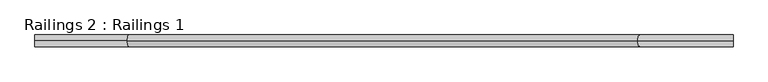
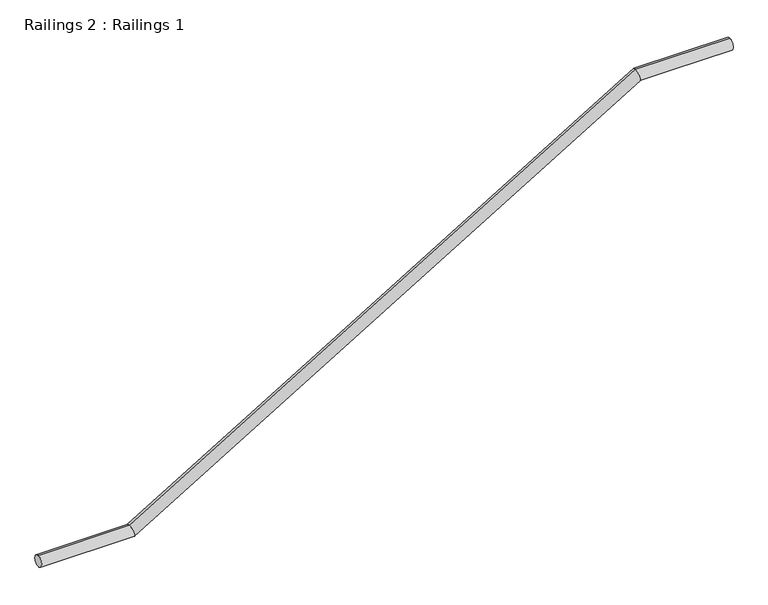
"""IFC4 building model written with IfcOpenShell, lengths in millimetres: railing geometry, Railings 2 : Railings 1."""

import ifcopenshell
import ifcopenshell.guid

model = None  # the IFC model being written
_history = None  # IfcOwnerHistory: only IFC2X3 demands one
_inside = {}  # id of a spatial element -> (the spatial element, [elements in it])
_under = {}  # id of a project, library or spatial element -> (it, [spatial elements below it])
_declared = {}  # id of a project -> (the project, [libraries it declares])
_typed = {}  # id of a type object -> (the type object, [elements of that type])
_made_of = {}  # id of a material, layer set ... -> (it, [elements and type objects made of it])


def new_model(schema):
    """Start an empty IFC model of exactly this schema.

    Asked for "IFC4X3", IfcOpenShell would pick the latest addendum, in which some entities
    have other attributes; the version numbers below select the first issue.
    IFC2X3 requires an IfcOwnerHistory on every rooted entity: one is made here for all.
    """
    global model, _history
    if schema == "IFC4X3":
        model = ifcopenshell.file(schema_version=(4, 3, 0, 0))
    else:
        model = ifcopenshell.file(schema=schema)
    _inside.clear()
    _under.clear()
    _declared.clear()
    _typed.clear()
    _made_of.clear()
    _history = None
    if model.schema == "IFC2X3":
        org = make("IfcOrganization", Name="unknown")
        user = make(
            "IfcPersonAndOrganization",
            ThePerson=make("IfcPerson", FamilyName="unknown"),
            TheOrganization=org,
        )
        app = make(
            "IfcApplication",
            ApplicationDeveloper=org,
            Version="unknown",
            ApplicationFullName="unknown",
            ApplicationIdentifier="unknown",
        )
        _history = make(
            "IfcOwnerHistory",
            OwningUser=user,
            OwningApplication=app,
            ChangeAction="ADDED",
            CreationDate=0,
        )
    return model


def make(cls, **values):
    """One entity of the class cls with the attributes given. An attribute that is None is left unset."""
    return model.create_entity(
        cls, **{name: value for name, value in values.items() if value is not None}
    )


def rooted(cls, **values):
    """An entity with a GlobalId (a new one), such as an element, a storey or a relation."""
    return make(cls, GlobalId=ifcopenshell.guid.new(), OwnerHistory=_history, **values)


def si_unit(unit_type, name, prefix=None):
    """IfcSIUnit, for example si_unit("LENGTHUNIT", "METRE", prefix="MILLI")."""
    return make("IfcSIUnit", UnitType=unit_type, Prefix=prefix, Name=name)


def assignment(units):
    """IfcUnitAssignment: the units of a project."""
    return None if units is None else make("IfcUnitAssignment", Units=units)


def point(xyz):
    """IfcCartesianPoint."""
    return None if xyz is None else make("IfcCartesianPoint", Coordinates=xyz)


def direction(xyz):
    """IfcDirection."""
    return None if xyz is None else make("IfcDirection", DirectionRatios=xyz)


def frame(location, z_axis=None, x_axis=None):
    """IfcAxis2Placement3D, a coordinate frame: its origin and axes. An axis left out is left unset."""
    return make(
        "IfcAxis2Placement3D",
        Location=point(location),
        Axis=direction(z_axis),
        RefDirection=direction(x_axis),
    )


def origin():
    """The frame at (0, 0, 0) with its axes left unset."""
    return frame((0.0, 0.0, 0.0))


def place(relative_to, where):
    """IfcLocalPlacement: puts the frame where relative to a parent placement (None: the world)."""
    return make(
        "IfcLocalPlacement", PlacementRelTo=relative_to, RelativePlacement=where
    )


def context(
    kind, dimensions, precision=None, world=None, true_north=None, identifier=None
):
    """IfcGeometricRepresentationContext, for example the 3D "Model" context."""
    return make(
        "IfcGeometricRepresentationContext",
        ContextIdentifier=identifier,
        ContextType=kind,
        CoordinateSpaceDimension=dimensions,
        Precision=precision,
        WorldCoordinateSystem=world,
        TrueNorth=true_north,
    )


def project(units=None, contexts=None):
    """IfcProject with its units and contexts."""
    return rooted(
        "IfcProject",
        Name="project",
        RepresentationContexts=contexts,
        UnitsInContext=assignment(units),
    )


def spatial(cls, under=None, at=None, **own):
    """A site, building, storey or space (cls), placed at a placement, below another one or the project."""
    s = rooted(cls, ObjectPlacement=at, **own)
    if under is not None:
        _under.setdefault(under.id(), (under, []))[1].append(s)
    return s


def circle_curve(where, radius):
    """IfcCircle in the frame where."""
    return make("IfcCircle", Position=where, Radius=radius)


def ellipse_curve(where, semi_axis1, semi_axis2):
    """IfcEllipse in the frame where."""
    return make(
        "IfcEllipse", Position=where, SemiAxis1=semi_axis1, SemiAxis2=semi_axis2
    )


def shape(context_of_items, identifier, shape_type, items):
    """IfcShapeRepresentation: the items that make up one representation, for example the "Body"."""
    return make(
        "IfcShapeRepresentation",
        ContextOfItems=context_of_items,
        RepresentationIdentifier=identifier,
        RepresentationType=shape_type,
        Items=items,
    )


def source(mapping_origin, context_of_items, identifier, shape_type, items):
    """IfcRepresentationMap: a shape defined once, which mapped items show again and again."""
    return make(
        "IfcRepresentationMap",
        MappingOrigin=mapping_origin,
        MappedRepresentation=shape(context_of_items, identifier, shape_type, items),
    )


def transform(
    local_origin,
    x_axis=None,
    y_axis=None,
    z_axis=None,
    scale=None,
    scale2=None,
    scale3=None,
    uniform=True,
):
    """IfcCartesianTransformationOperator3D, or its non-uniform kind. x_axis, y_axis, z_axis: its Axis1, 2, 3."""
    if uniform:
        return make(
            "IfcCartesianTransformationOperator3D",
            Axis1=direction(x_axis),
            Axis2=direction(y_axis),
            LocalOrigin=point(local_origin),
            Scale=scale,
            Axis3=direction(z_axis),
        )
    return make(
        "IfcCartesianTransformationOperator3DnonUniform",
        Axis1=direction(x_axis),
        Axis2=direction(y_axis),
        LocalOrigin=point(local_origin),
        Scale=scale,
        Axis3=direction(z_axis),
        Scale2=scale2,
        Scale3=scale3,
    )


def mapped(mapping_source, mapping_target):
    """IfcMappedItem: shows the shape of a source again, moved by a transform."""
    return make(
        "IfcMappedItem", MappingSource=mapping_source, MappingTarget=mapping_target
    )


def made_of(thing, what):
    """Note that an element or type object is made of a material, layer set ...; save() writes the relation."""
    if what is not None:
        _made_of.setdefault(what.id(), (what, []))[1].append(thing)
    return thing


def element(
    cls,
    number,
    at=None,
    inside=None,
    cuts=None,
    type_object=None,
    material=None,
    context=None,
    identifier="Body",
    shape_type=None,
    held_by="IfcProductDefinitionShape",
    body=None,
    shapes=None,
    **own,
):
    """One element of the class cls, such as IfcWall. Its Tag is "e" and its number.

    at: its placement. inside: the storey or other place that contains it. cuts: it is an
    opening in that element (IfcRelVoidsElement). A single representation is given by context,
    identifier, shape_type and body (its items); several are given by shapes. held_by: the class
    of the entity that holds the representations. save() writes the other relations.
    """
    e = rooted(cls, Tag="e%d" % number, ObjectPlacement=at, **own)
    if body is not None:
        shapes = [shape(context, identifier, shape_type, body)]
    if shapes is not None:
        e.Representation = make(held_by, Representations=shapes)
    if inside is not None:
        _inside.setdefault(inside.id(), (inside, []))[1].append(e)
    if cuts is not None:
        rooted(
            "IfcRelVoidsElement", RelatingBuildingElement=cuts, RelatedOpeningElement=e
        )
    if type_object is not None:
        _typed.setdefault(type_object.id(), (type_object, []))[1].append(e)
    return made_of(e, material)


def aggregate(whole, parts):
    """IfcRelAggregates: a whole, such as a stair, and the parts it consists of."""
    return rooted("IfcRelAggregates", RelatingObject=whole, RelatedObjects=parts)


def save(model, path):
    """Write the relations noted so far, then the file.

    IfcRelAggregates (storeys below a building ...), IfcRelContainedInSpatialStructure (elements
    in a storey), IfcRelDefinesByType, IfcRelAssociatesMaterial and IfcRelDeclares: one each for
    every whole, place, type object, material and project.
    """
    for whole, parts in _under.values():
        aggregate(whole, parts)
    for where, things in _inside.values():
        rooted(
            "IfcRelContainedInSpatialStructure",
            RelatedElements=things,
            RelatingStructure=where,
        )
    for kind, things in _typed.values():
        rooted("IfcRelDefinesByType", RelatedObjects=things, RelatingType=kind)
    for what, things in _made_of.values():
        rooted("IfcRelAssociatesMaterial", RelatedObjects=things, RelatingMaterial=what)
    for by, libraries in _declared.values():
        rooted("IfcRelDeclares", RelatingContext=by, RelatedDefinitions=libraries)
    model.write(path)


def plane_surface(at):
    """IfcPlane: the flat surface through the origin of the frame at, square to its z axis."""
    return make("IfcPlane", Position=at)


def cylinder_surface(at, radius):
    """IfcCylindricalSurface: all points at the distance radius from the z axis of the frame at."""
    return make("IfcCylindricalSurface", Position=at, Radius=radius)


def advanced_brep(points, edges, surfaces, faces):
    """IfcAdvancedBrep: a solid bounded by faces that lie on surfaces and meet in shared edges.

    An edge is (start, end): straight between two places in points (the first is 0);
    or (start, end, curve); or (start, end, curve, False) where it runs against its curve.
    A face is (place in surfaces, loops), or (place, loops, False) where it looks against
    its surface's normal. A loop lists edges by number (the first is 1), with a minus sign
    where the edge is run from its end to its start. The first loop is the outer one.
    """
    corners = [point(p) for p in points]
    vertices = [make("IfcVertexPoint", VertexGeometry=c) for c in corners]
    made = []
    for start, end, *more in edges:
        made.append(
            make(
                "IfcEdgeCurve",
                EdgeStart=vertices[start],
                EdgeEnd=vertices[end],
                EdgeGeometry=more[0] if more else make("IfcPolyline", Points=[corners[start], corners[end]]),
                SameSense=more[1] if len(more) > 1 else True,
            )
        )
    hull = []
    for where, loops, *sense in faces:
        bounds = []
        for j, loop in enumerate(loops):
            ring = [make("IfcOrientedEdge", EdgeElement=made[abs(k) - 1], Orientation=k > 0) for k in loop]
            bounds.append(
                make(
                    "IfcFaceOuterBound" if j == 0 else "IfcFaceBound",
                    Bound=make("IfcEdgeLoop", EdgeList=ring),
                    Orientation=True,
                )
            )
        hull.append(make("IfcAdvancedFace", Bounds=bounds, FaceSurface=surfaces[where], SameSense=sense[0] if sense else True))
    return make("IfcAdvancedBrep", Outer=make("IfcClosedShell", CfsFaces=hull))


def railings_2_railings_1_8e6ca935(model_context):
    return source(origin(), model_context, "Body", "AdvancedBrep", [
        advanced_brep(
        [(27576.4590778, 25902.7078032, 267263.8511364), (27576.4590778, 25902.7078032, 267301.9511364), (25613.2527478, 25902.7078032, 266261.85), (25602.6654079, 25902.7078032, 266299.95), (25303.1590778, 25902.7078032, 266299.95), (25303.1590778, 25902.7078032, 266261.85), (27276.9527478, 25902.7078032, 267263.8511364), (27266.3654079, 25902.7078032, 267301.9511364)],
        [
            (0, 1, circle_curve(frame((27576.4590778, 25902.7078032, 267282.9011364), z_axis=(1.0, 0.0, 0.0), x_axis=(0.0, 0.0, 1.0)), 19.05)),
            (1, 0, circle_curve(frame((27576.4590778, 25902.7078032, 267282.9011364), z_axis=(1.0, 0.0, 0.0), x_axis=(0.0, 0.0, 1.0)), 19.05)),
            (2, 3, ellipse_curve(frame((25607.9590778, 25902.7078032, 266280.9), z_axis=(-0.9634917766912359, 0.0, -0.2677379245612505), x_axis=(0.2677379245612497, 0.0, -0.9634917766912361)), 19.7718346, 19.05)),
            (3, 4),
            (4, 5, circle_curve(frame((25303.1590778, 25902.7078032, 266280.9), z_axis=(1.0, 0.0, 0.0), x_axis=(0.0, 0.0, 1.0)), 19.05)),
            (5, 2),
            (3, 2, ellipse_curve(frame((25607.9590778, 25902.7078032, 266280.9), z_axis=(-0.9634917766912359, 0.0, -0.2677379245612505), x_axis=(0.2677379245612497, 0.0, -0.9634917766912361)), 19.7718346, 19.05)),
            (5, 4, circle_curve(frame((25303.1590778, 25902.7078032, 266280.9), z_axis=(1.0, 0.0, 0.0), x_axis=(0.0, 0.0, 1.0)), 19.05)),
            (0, 6),
            (6, 7, ellipse_curve(frame((27271.6590778, 25902.7078032, 267282.9011364), z_axis=(0.9634917766912359, 0.0, 0.2677379245612505), x_axis=(0.2677379245612497, 0.0, -0.9634917766912361)), 19.7718346, 19.05)),
            (7, 1),
            (7, 6, ellipse_curve(frame((27271.6590778, 25902.7078032, 267282.9011364), z_axis=(0.9634917766912359, 0.0, 0.2677379245612505), x_axis=(0.2677379245612497, 0.0, -0.9634917766912361)), 19.7718346, 19.05)),
            (6, 2),
            (3, 7),
        ],
        [
            plane_surface(frame((27576.4590778, 25883.6578032, 267282.9011364), z_axis=(1.0, 0.0, 0.0), x_axis=(0.0, -1.0, 0.0))),
            cylinder_surface(frame((25607.9590778, 25902.7078032, 266280.9), z_axis=(1.0, 0.0, 0.0), x_axis=(0.0, 0.0, 1.0)), 19.05),
            plane_surface(frame((25303.1590778, 25883.6578032, 266280.9), z_axis=(-1.0, 0.0, 0.0), x_axis=(0.0, -1.0, 0.0))),
            cylinder_surface(frame((27576.4590778, 25902.7078032, 267282.9011364), z_axis=(1.0, 0.0, 0.0), x_axis=(0.0, 0.0, 1.0)), 19.05),
            cylinder_surface(frame((27271.6590778, 25902.7078032, 267282.9011364), z_axis=(0.8566328075032683, 0.0, 0.5159265772462865), x_axis=(-0.5159265772462865, 0.0, 0.8566328075032683)), 19.05),
        ],
        [
            (0, [[1, 2]]),
            (1, [[3, 4, 5, 6]]),
            (1, [[7, -6, 8, -4]]),
            (2, [[-5, -8]]),
            (3, [[-1, 9, 10, 11]]),
            (3, [[-2, -11, 12, -9]]),
            (4, [[-10, 13, -7, 14]]),
            (4, [[-12, -14, -3, -13]]),
        ],
    ),
    ])


if __name__ == "__main__":
    model = new_model("IFC4")
    model_context = context("Model", 3, world=origin())
    ifc_project = project(units=[si_unit("LENGTHUNIT", "METRE", prefix="MILLI")], contexts=[model_context])
    site = spatial("IfcSite", under=ifc_project)
    building = spatial("IfcBuilding", under=site)
    placement = place(None, origin())
    railings_2_railings_1_shape = railings_2_railings_1_8e6ca935(model_context)
    element("IfcRailing", 1, ObjectType="Railings 2 : Railings 1", at=placement, inside=building, context=model_context, shape_type="MappedRepresentation", body=[
        mapped(railings_2_railings_1_shape, transform((0.0, 0.0, 0.0), x_axis=(1.0, 0.0, 0.0), y_axis=(0.0, 1.0, 0.0), z_axis=(0.0, 0.0, 1.0))),
    ])
    save(model, "model.ifc")

# Revit data of these elements
# Element 1 (IfcRailing, "Railings 2 : Railings 1")
#   Materials on its faces: "ALUM. RAILING"
# Materials
#   "ALUM. RAILING": class "Generic", colour RGB 255 255 255, transparency 0, Cost = 0
